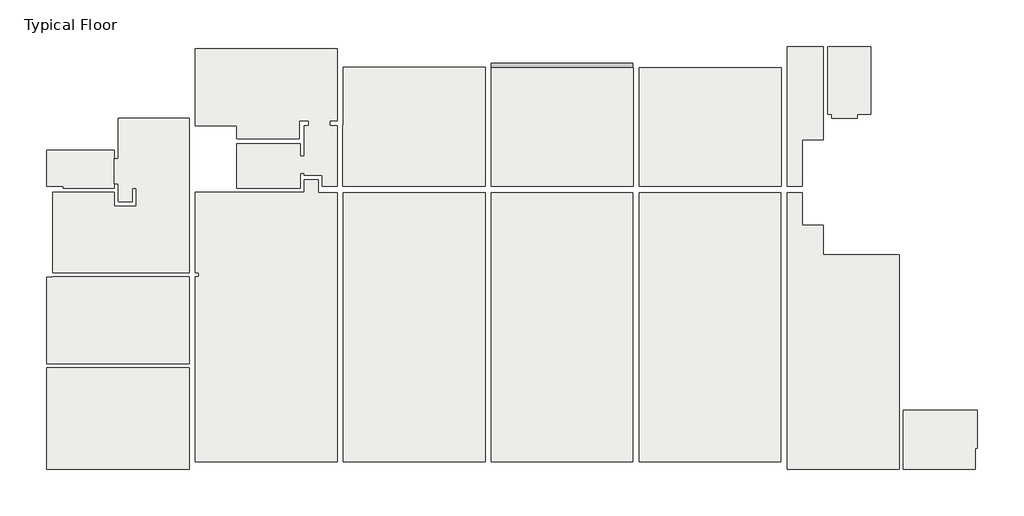
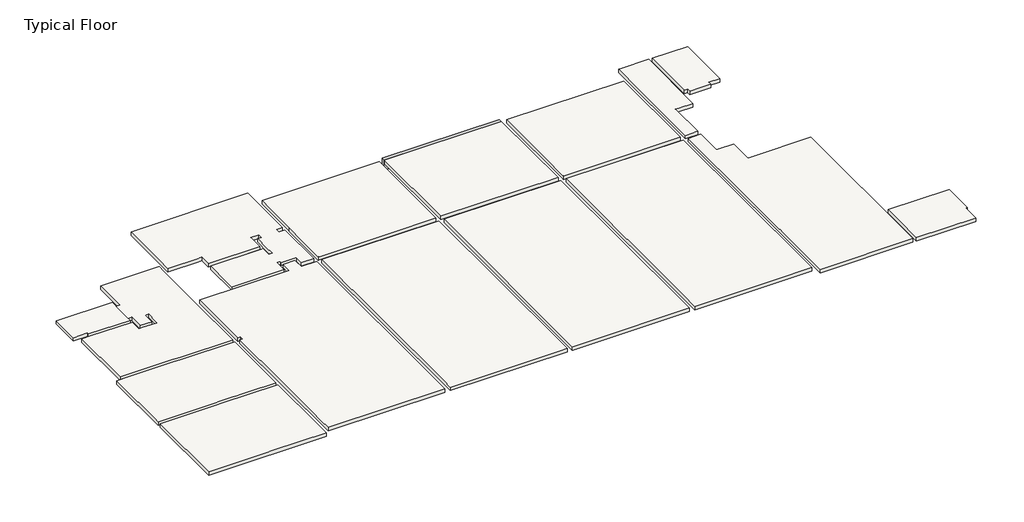
# One storey: 16 slabs, 1 beam.
"""IFC4 building model written with IfcOpenShell, lengths in millimetres."""

from ifc_helpers import new_model, si_unit, frame, origin, place, context, project, spatial, polyline, outline, extrude, faceted_brep, element, save

model = new_model("IFC4")

# Units and contexts
model_context = context("Model", 3, world=origin())
ifc_project = project(units=[si_unit("LENGTHUNIT", "METRE", prefix="MILLI")], contexts=[model_context])

# Site, building, storey
site = spatial("IfcSite", under=ifc_project)
building = spatial("IfcBuilding", under=site)
storey = spatial("IfcBuildingStorey", under=building, Name="Typical Floor", Elevation=4000.0)

# Beam
placement = place(None, origin())
element("IfcBeam", 1, ObjectType="Concrete Rectengular Beam : 20/60", at=placement, inside=storey, context=model_context, shape_type="Brep", body=[
    faceted_brep([(7056.7343244, 23405.5571184, 4000.0), (358.2285773, 23405.5571184, 4000.0), (358.2285773, 23210.5571184, 4000.0), (7056.7343244, 23210.5571184, 4000.0), (7056.7343244, 23405.5571184, 3400.0), (358.2285773, 23405.5571184, 3400.0), (7056.7343244, 23205.5571184, 3400.0), (358.2285773, 23205.5571184, 3400.0), (7056.7343244, 23205.5571184, 3790.0), (358.2285773, 23205.5571184, 3790.0), (7056.7343244, 23210.5571184, 3790.0), (7056.7343244, 23206.5724441, 3790.0), (358.2285773, 23206.5724441, 3790.0), (358.2285773, 23210.5571184, 3790.0)], [[[0, 1, 2, 3]], [[0, 4, 5, 1]], [[4, 6, 7, 5]], [[7, 6, 8, 9]], [[4, 0, 3, 10, 11, 8, 6]], [[1, 5, 7, 9, 12, 13, 2]], [[10, 13, 12, 9, 8, 11]], [[13, 10, 3, 2]]]),
])

# Slabs
element("IfcSlab", 2, ObjectType="21", at=placement, inside=storey, context=model_context, shape_type="Brep", body=[
    faceted_brep([(-6644.3384725, 23225.5571184, 3790.0), (58.2285773, 23225.5571184, 3790.0), (58.2285773, 23206.5724441, 3790.0), (68.2285773, 23206.5724441, 3790.0), (68.2285773, 17597.4228975, 3790.0), (58.2285773, 17597.4228975, 3790.0), (58.2285773, 17587.4228975, 3790.0), (-6644.3384725, 17587.4228975, 3790.0), (-6644.3384725, 17597.4228975, 3790.0), (-6674.3384725, 17597.4228975, 3790.0), (-6674.3384725, 20454.6567352, 3790.0), (-6644.3384725, 20454.6567352, 3790.0), (-6644.3384725, 23205.5571184, 3790.0), (58.2285773, 23225.5571184, 4000.0), (-6644.3384725, 23225.5571184, 4000.0), (-6644.3384725, 20704.6567352, 4000.0), (-6644.3384725, 20454.6567352, 4000.0), (-6674.3384725, 20454.6567352, 4000.0), (-6674.3384725, 17597.4228975, 4000.0), (-6644.3384725, 17597.4228975, 4000.0), (-6644.3384725, 17587.4228975, 4000.0), (58.2285773, 17587.4228975, 4000.0), (58.2285773, 17597.4228975, 4000.0), (68.2285773, 17597.4228975, 4000.0), (68.2285773, 23206.5724441, 4000.0), (58.2285773, 23206.5724441, 4000.0)], [[[0, 1, 2, 3, 4, 5, 6, 7, 8, 9, 10, 11, 12]], [[13, 14, 15, 16, 17, 18, 19, 20, 21, 22, 23, 24, 25]], [[3, 24, 23, 4]], [[6, 21, 20, 7]], [[17, 10, 9, 18]], [[0, 14, 13, 1]], [[14, 0, 12, 11, 16, 15]], [[2, 25, 24, 3]], [[25, 2, 1, 13]], [[5, 22, 21, 6]], [[22, 5, 4, 23]], [[16, 11, 10, 17]], [[8, 19, 18, 9]], [[19, 8, 7, 20]]]),
])
element("IfcSlab", 3, ObjectType="21", at=placement, inside=storey, context=model_context, shape_type="Brep", body=[
    faceted_brep([(7061.7343244, 17597.4228975, 3790.0), (7056.7343244, 17597.4228975, 3790.0), (358.2285773, 17597.4228975, 3790.0), (353.2285773, 17597.4228975, 3790.0), (353.2285773, 23206.5724441, 3790.0), (358.2285773, 23206.5724441, 3790.0), (358.2285773, 23210.5571184, 3790.0), (7056.7343244, 23210.5571184, 3790.0), (7056.7343244, 23206.5724441, 3790.0), (7061.7343244, 23206.5724441, 3790.0), (353.2285773, 17597.4228975, 4000.0), (358.2285773, 17597.4228975, 4000.0), (7056.7343244, 17597.4228975, 4000.0), (7061.7343244, 17597.4228975, 4000.0), (7061.7343244, 23206.5724441, 4000.0), (7056.7343244, 23206.5724441, 4000.0), (7056.7343244, 23210.5571184, 4000.0), (358.2285773, 23210.5571184, 4000.0), (358.2285773, 23206.5724441, 4000.0), (353.2285773, 23206.5724441, 4000.0)], [[[0, 1, 2, 3, 4, 5, 6, 7, 8, 9]], [[10, 11, 12, 13, 14, 15, 16, 17, 18, 19]], [[13, 0, 9, 14]], [[3, 2, 1, 0, 13, 12, 11, 10]], [[3, 10, 19, 4]], [[6, 17, 16, 7]], [[5, 18, 17, 6]], [[18, 5, 4, 19]], [[8, 15, 14, 9]], [[15, 8, 7, 16]]]),
])
element("IfcSlab", 4, ObjectType="21", at=placement, inside=storey, context=model_context, shape_type="Brep", body=[
    faceted_brep([(7356.7343244, 23206.5724441, 3790.0), (7356.7343244, 23210.5571184, 3790.0), (14058.5350907, 23210.5571184, 3790.0), (14058.5350907, 23206.5724441, 3790.0), (14063.5350907, 23206.5724441, 3790.0), (14063.5350907, 23205.5571184, 3790.0), (14063.5350907, 17597.4228975, 3790.0), (14058.5350907, 17597.4228975, 3790.0), (14058.5350907, 17587.4228975, 3790.0), (7356.7343244, 17587.4228975, 3790.0), (7356.7343244, 17597.4228975, 3790.0), (7351.7343244, 17597.4228975, 3790.0), (7351.7343244, 23206.5724441, 3790.0), (7356.7343244, 23210.5571184, 4000.0), (7356.7343244, 23206.5724441, 4000.0), (7351.7343244, 23206.5724441, 4000.0), (7351.7343244, 17597.4228975, 4000.0), (7356.7343244, 17597.4228975, 4000.0), (7356.7343244, 17587.4228975, 4000.0), (14058.5350907, 17587.4228975, 4000.0), (14058.5350907, 17597.4228975, 4000.0), (14063.5350907, 17597.4228975, 4000.0), (14063.5350907, 23205.5571184, 4000.0), (14063.5350907, 23206.5724441, 4000.0), (14058.5350907, 23206.5724441, 4000.0), (14058.5350907, 23210.5571184, 4000.0)], [[[0, 1, 2, 3, 4, 5, 6, 7, 8, 9, 10, 11, 12]], [[13, 14, 15, 16, 17, 18, 19, 20, 21, 22, 23, 24, 25]], [[4, 23, 22, 21, 6, 5]], [[18, 9, 8, 19]], [[15, 12, 11, 16]], [[1, 13, 25, 2]], [[0, 14, 13, 1]], [[14, 0, 12, 15]], [[17, 10, 9, 18]], [[10, 17, 16, 11]], [[24, 3, 2, 25]], [[3, 24, 23, 4]], [[20, 7, 6, 21]], [[7, 20, 19, 8]]]),
])
element("IfcSlab", 5, ObjectType="21", at=placement, inside=storey, context=model_context, shape_type="Brep", body=[
    faceted_brep([(14058.5350907, 17297.4228975, 3790.0), (14058.5350907, 4552.8176548, 3790.0), (7356.7343244, 4552.8176548, 3790.0), (7356.7343244, 17297.4228975, 3790.0), (14058.5350907, 17297.4228975, 4000.0), (7356.7343244, 17297.4228975, 4000.0), (7356.7343244, 5204.8099919, 4000.0), (7356.7343244, 4552.8176548, 4000.0), (14058.5350907, 4552.8176548, 4000.0), (14058.5350907, 5204.8099919, 4000.0)], [[[0, 1, 2, 3]], [[4, 5, 6, 7, 8, 9]], [[1, 0, 4, 9, 8]], [[2, 1, 8, 7]], [[3, 2, 7, 6, 5]], [[0, 3, 5, 4]]]),
])
element("IfcSlab", 6, ObjectType="21", at=placement, inside=storey, context=model_context, shape_type="Brep", body=[
    faceted_brep([(7056.7343244, 17297.4228975, 3790.0), (7056.7343244, 4552.8176548, 3790.0), (358.2285773, 4552.8176548, 3790.0), (358.2285773, 17297.4228975, 3790.0), (7056.7343244, 17297.4228975, 4000.0), (358.2285773, 17297.4228975, 4000.0), (358.2285773, 5204.8099919, 4000.0), (358.2285773, 4552.8176548, 4000.0), (7056.7343244, 4552.8176548, 4000.0), (7056.7343244, 5204.8099919, 4000.0)], [[[0, 1, 2, 3]], [[4, 5, 6, 7, 8, 9]], [[1, 0, 4, 9, 8]], [[2, 1, 8, 7]], [[3, 2, 7, 6, 5]], [[0, 3, 5, 4]]]),
])
element("IfcSlab", 7, ObjectType="21", at=placement, inside=storey, context=model_context, shape_type="Brep", body=[
    faceted_brep([(58.2285773, 17297.4228975, 3790.0), (58.2285773, 4552.8176548, 3790.0), (-6644.3384725, 4552.8176548, 3790.0), (-6644.3384725, 17297.4228975, 3790.0), (58.2285773, 17297.4228975, 4000.0), (-6644.3384725, 17297.4228975, 4000.0), (-6644.3384725, 5204.8099919, 4000.0), (-6644.3384725, 4552.8176548, 4000.0), (58.2285773, 4552.8176548, 4000.0), (58.2285773, 5204.8099919, 4000.0)], [[[0, 1, 2, 3]], [[4, 5, 6, 7, 8, 9]], [[1, 0, 4, 9, 8]], [[2, 1, 8, 7]], [[3, 2, 7, 6, 5]], [[0, 3, 5, 4]]]),
])
element("IfcSlab", 8, ObjectType="21", at=placement, inside=storey, context=model_context, shape_type="Brep", body=[
    faceted_brep([(-13943.2656756, 9206.6873866, 3790.0), (-20690.7944112, 9206.6873866, 3790.0), (-20690.7944112, 13148.3800933, 3790.0), (-20690.7944112, 13298.3800933, 3790.0), (-20386.1465057, 13298.5145478, 3790.0), (-20386.1465057, 13303.9096088, 3790.0), (-20386.1465057, 13308.9096088, 3790.0), (-17368.3423039, 13308.9096088, 3790.0), (-17368.3423039, 13303.9096088, 3790.0), (-16968.3423039, 13303.9096088, 3790.0), (-16968.3423039, 13308.9096088, 3790.0), (-13944.4917292, 13308.9096088, 3790.0), (-13944.4917292, 13303.9096088, 3790.0), (-13943.2656756, 13303.9096088, 3790.0), (-20690.7944112, 9206.6873866, 4000.0), (-20678.0944112, 9206.6873866, 4000.0), (-17516.5223806, 9206.6873866, 4000.0), (-17116.5223806, 9206.6873866, 4000.0), (-13943.2656756, 9206.6873866, 4000.0), (-13943.2656756, 13303.9096088, 4000.0), (-13944.4917292, 13303.9096088, 4000.0), (-13944.4917292, 13308.9096088, 4000.0), (-16968.3423039, 13308.9096088, 4000.0), (-16968.3423039, 13303.9096088, 4000.0), (-17368.3423039, 13303.9096088, 4000.0), (-17368.3423039, 13308.9096088, 4000.0), (-20386.1465057, 13308.9096088, 4000.0), (-20386.1465057, 13298.5145478, 4000.0), (-20540.7944404, 13298.4462949, 4000.0), (-20690.7944112, 13298.3800933, 4000.0), (-20690.7944112, 13148.3800933, 4000.0)], [[[0, 1, 2, 3, 4, 5, 6, 7, 8, 9, 10, 11, 12, 13]], [[14, 15, 16, 17, 18, 19, 20, 21, 22, 23, 24, 25, 26, 27, 28, 29, 30]], [[18, 0, 13, 19]], [[1, 0, 18, 17, 16, 15, 14]], [[1, 14, 30, 29, 3, 2]], [[6, 26, 25, 7]], [[10, 22, 21, 11]], [[3, 29, 28, 27, 4]], [[4, 27, 26, 6, 5]], [[9, 23, 22, 10]], [[23, 9, 8, 24]], [[24, 8, 7, 25]], [[12, 20, 19, 13]], [[20, 12, 11, 21]]]),
])
element("IfcSlab", 9, ObjectType="21", at=placement, inside=storey, context=model_context, shape_type="Brep", body=[
    faceted_brep([(-13943.2656756, 9006.6873866, 3790.0), (-13943.2656756, 4206.6682295, 3790.0), (-20492.8250626, 4206.6682295, 3790.0), (-20690.7944112, 4206.6682295, 3790.0), (-20690.7944112, 9006.6873866, 3790.0), (-13943.2656756, 4206.6682295, 4000.0), (-13943.2656756, 5204.8099919, 4000.0), (-13943.2656756, 9006.6873866, 4000.0), (-17116.5223806, 9006.6873866, 4000.0), (-17516.5223806, 9006.6873866, 4000.0), (-20678.0944112, 9006.6873866, 4000.0), (-20690.7944112, 9006.6873866, 4000.0), (-20690.7944112, 8705.6720609, 4000.0), (-20690.7944112, 4206.6682295, 4000.0), (-20492.8250626, 4206.6682295, 4000.0), (-17416.9438365, 4206.6682295, 4000.0), (-17016.9438365, 4206.6682295, 4000.0)], [[[0, 1, 2, 3, 4]], [[5, 6, 7, 8, 9, 10, 11, 12, 13, 14, 15, 16]], [[1, 0, 7, 6, 5]], [[1, 5, 16, 15, 14, 13, 3, 2]], [[4, 3, 13, 12, 11]], [[0, 4, 11, 10, 9, 8, 7]]]),
])
element("IfcSlab", 10, ObjectType="21", at=placement, inside=storey, context=model_context, shape_type="Brep", body=[
    faceted_brep([(-8494.4725721, 17905.9594172, 3790.0), (-7834.4725721, 17905.9594172, 3790.0), (-7834.4725721, 17297.4228975, 3790.0), (-7634.4725721, 17297.4228975, 3790.0), (-6944.3384725, 17297.4228975, 3790.0), (-6944.3384725, 4552.8176548, 3790.0), (-13643.2656756, 4552.8176548, 3790.0), (-13643.2656756, 13303.9096088, 3790.0), (-13494.4917292, 13303.9096088, 3790.0), (-13494.4917292, 13503.9096088, 3790.0), (-13643.2656756, 13503.9096088, 3790.0), (-13643.2656756, 17304.7716778, 3790.0), (-8494.4725721, 17304.7716778, 3790.0), (-8494.4725721, 17504.7716778, 3790.0), (-7834.4725721, 17905.9594172, 4000.0), (-8494.4725721, 17905.9594172, 4000.0), (-8494.4725721, 17504.7716778, 4000.0), (-8494.4725721, 17304.7716778, 4000.0), (-13643.2656756, 17304.7716778, 4000.0), (-13643.2656756, 13503.9096088, 4000.0), (-13494.4917292, 13503.9096088, 4000.0), (-13494.4917292, 13303.9096088, 4000.0), (-13643.2656756, 13303.9096088, 4000.0), (-13643.2656756, 9206.6873866, 4000.0), (-13643.2656756, 9006.6873866, 4000.0), (-13643.2656756, 5204.8099919, 4000.0), (-13643.2656756, 4552.8176548, 4000.0), (-6944.3384725, 4552.8176548, 4000.0), (-6944.3384725, 5204.8099919, 4000.0), (-6944.3384725, 17297.4228975, 4000.0), (-7634.4725721, 17297.4228975, 4000.0), (-7834.4725721, 17297.4228975, 4000.0)], [[[0, 1, 2, 3, 4, 5, 6, 7, 8, 9, 10, 11, 12, 13]], [[14, 15, 16, 17, 18, 19, 20, 21, 22, 23, 24, 25, 26, 27, 28, 29, 30, 31]], [[15, 0, 13, 12, 17, 16]], [[1, 0, 15, 14]], [[2, 1, 14, 31]], [[2, 31, 30, 29, 4, 3]], [[5, 4, 29, 28, 27]], [[6, 5, 27, 26]], [[7, 6, 26, 25, 24, 23, 22]], [[8, 7, 22, 21]], [[9, 8, 21, 20]], [[10, 9, 20, 19]], [[11, 10, 19, 18]], [[12, 11, 18, 17]]]),
])
element("IfcSlab", 11, ObjectType="21", at=placement, inside=storey, context=model_context, shape_type="Brep", body=[
    faceted_brep([(-8685.7944112, 19594.6567352, 3790.0), (-8685.7944112, 19006.7257008, 3790.0), (-8485.7944112, 19006.7257008, 3790.0), (-8485.7944112, 19594.6567352, 3790.0), (-8485.7944112, 20454.6567352, 3790.0), (-8291.2541813, 20454.6567352, 3790.0), (-8291.2541813, 20704.6567352, 3790.0), (-8735.7944112, 20704.6567352, 3790.0), (-8735.7944112, 20454.6567352, 3790.0), (-8735.7944112, 19844.6567352, 3790.0), (-11690.9285108, 19844.6567352, 3790.0), (-11690.9285108, 20459.7142065, 3790.0), (-11890.9285108, 20459.7142065, 3790.0), (-13643.2656756, 20459.7142065, 3790.0), (-13643.2656756, 24104.7142065, 3790.0), (-6944.3384725, 24104.7142065, 3790.0), (-6944.3384725, 20704.6567352, 3790.0), (-7292.0970932, 20704.6567352, 3790.0), (-7292.0970932, 20454.6567352, 3790.0), (-6944.3384725, 20454.6567352, 3790.0), (-6944.3384725, 17597.4228975, 3790.0), (-7634.4725721, 17597.4228975, 3790.0), (-7634.4725721, 17905.9594172, 3790.0), (-7634.4725721, 18105.9594172, 3790.0), (-8494.4725721, 18105.9594172, 3790.0), (-8494.4725721, 18206.553287, 3790.0), (-8694.4725721, 18206.553287, 3790.0), (-8694.4725721, 17504.7716778, 3790.0), (-11690.9285108, 17504.7716778, 3790.0), (-11690.9285108, 19594.6567352, 3790.0), (-8735.7944112, 19594.6567352, 3790.0), (-8685.7944112, 19006.7257008, 4000.0), (-8685.7944112, 19594.6567352, 4000.0), (-8735.7944112, 19594.6567352, 4000.0), (-11690.9285108, 19594.6567352, 4000.0), (-11690.9285108, 17504.7716778, 4000.0), (-8694.4725721, 17504.7716778, 4000.0), (-8694.4725721, 18206.553287, 4000.0), (-8494.4725721, 18206.553287, 4000.0), (-8494.4725721, 18105.9594172, 4000.0), (-7634.4725721, 18105.9594172, 4000.0), (-7634.4725721, 17905.9594172, 4000.0), (-7634.4725721, 17597.4228975, 4000.0), (-6944.3384725, 17597.4228975, 4000.0), (-6944.3384725, 20454.6567352, 4000.0), (-7292.0970932, 20454.6567352, 4000.0), (-7292.0970932, 20704.6567352, 4000.0), (-6944.3384725, 20704.6567352, 4000.0), (-6944.3384725, 24104.7142065, 4000.0), (-13643.2656756, 24104.7142065, 4000.0), (-13643.2656756, 20459.7142065, 4000.0), (-11890.9285108, 20459.7142065, 4000.0), (-11690.9285108, 20459.7142065, 4000.0), (-11690.9285108, 19844.6567352, 4000.0), (-8735.7944112, 19844.6567352, 4000.0), (-8735.7944112, 20454.6567352, 4000.0), (-8735.7944112, 20704.6567352, 4000.0), (-8291.2541813, 20704.6567352, 4000.0), (-8291.2541813, 20454.6567352, 4000.0), (-8485.7944112, 20454.6567352, 4000.0), (-8485.7944112, 19594.6567352, 4000.0), (-8485.7944112, 19006.7257008, 4000.0)], [[[0, 1, 2, 3, 4, 5, 6, 7, 8, 9, 10, 11, 12, 13, 14, 15, 16, 17, 18, 19, 20, 21, 22, 23, 24, 25, 26, 27, 28, 29, 30]], [[31, 32, 33, 34, 35, 36, 37, 38, 39, 40, 41, 42, 43, 44, 45, 46, 47, 48, 49, 50, 51, 52, 53, 54, 55, 56, 57, 58, 59, 60, 61]], [[32, 0, 30, 29, 34, 33]], [[1, 0, 32, 31]], [[2, 1, 31, 61]], [[2, 61, 60, 59, 4, 3]], [[5, 4, 59, 58]], [[6, 5, 58, 57]], [[7, 6, 57, 56]], [[7, 56, 55, 54, 9, 8]], [[10, 9, 54, 53]], [[11, 10, 53, 52]], [[11, 52, 51, 50, 13, 12]], [[14, 13, 50, 49]], [[15, 14, 49, 48]], [[16, 15, 48, 47]], [[17, 16, 47, 46]], [[18, 17, 46, 45]], [[19, 18, 45, 44]], [[20, 19, 44, 43]], [[21, 20, 43, 42]], [[21, 42, 41, 40, 23, 22]], [[24, 23, 40, 39]], [[25, 24, 39, 38]], [[26, 25, 38, 37]], [[27, 26, 37, 36]], [[28, 27, 36, 35]], [[29, 28, 35, 34]]]),
])
element("IfcSlab", 12, ObjectType="21", at=placement, inside=storey, context=model_context, shape_type="Brep", body=[
    faceted_brep([(-17492.1354074, 18905.1165054, 3790.0), (-17292.1354074, 18905.1165054, 3790.0), (-17292.1354074, 20806.0552027, 3790.0), (-13943.2656756, 20806.0552027, 3790.0), (-13943.2656756, 13503.9096088, 3790.0), (-20386.1465057, 13503.9096088, 3790.0), (-20386.1465057, 17305.3655475, 3790.0), (-19891.6373231, 17305.3655475, 3790.0), (-19891.6373231, 17304.7716778, 3790.0), (-17492.1354074, 17304.7716778, 3790.0), (-17492.1354074, 16652.7793406, 3790.0), (-17292.1354074, 16652.7793406, 3790.0), (-16441.1583959, 16652.7793406, 3790.0), (-16441.1583959, 16852.7793406, 3790.0), (-16441.1583959, 17503.7563521, 3790.0), (-16641.1583959, 17503.7563521, 3790.0), (-16641.1583959, 16852.7793406, 3790.0), (-17292.1354074, 16852.7793406, 3790.0), (-17292.1354074, 17706.9747429, 3790.0), (-17492.1354074, 17706.9747429, 3790.0), (-17292.1354074, 18905.1165054, 4000.0), (-17492.1354074, 18905.1165054, 4000.0), (-17492.1354074, 17706.9747429, 4000.0), (-17292.1354074, 17706.9747429, 4000.0), (-17292.1354074, 16852.7793406, 4000.0), (-16641.1583959, 16852.7793406, 4000.0), (-16641.1583959, 17503.7563521, 4000.0), (-16441.1583959, 17503.7563521, 4000.0), (-16441.1583959, 16852.7793406, 4000.0), (-16441.1583959, 16652.7793406, 4000.0), (-17292.1354074, 16652.7793406, 4000.0), (-17492.1354074, 16652.7793406, 4000.0), (-17492.1354074, 17304.7716778, 4000.0), (-19891.6373231, 17304.7716778, 4000.0), (-19891.6373231, 17305.3655475, 4000.0), (-20386.1465057, 17305.3655475, 4000.0), (-20386.1465057, 13648.5145478, 4000.0), (-20386.1465057, 13503.9096088, 4000.0), (-17368.3423039, 13503.9096088, 4000.0), (-16968.3423039, 13503.9096088, 4000.0), (-13944.4917292, 13503.9096088, 4000.0), (-13943.2656756, 13503.9096088, 4000.0), (-13943.2656756, 17304.7716778, 4000.0), (-13943.2656756, 20334.7142065, 4000.0), (-13943.2656756, 20806.0552027, 4000.0), (-17292.1354074, 20806.0552027, 4000.0)], [[[0, 1, 2, 3, 4, 5, 6, 7, 8, 9, 10, 11, 12, 13, 14, 15, 16, 17, 18, 19]], [[20, 21, 22, 23, 24, 25, 26, 27, 28, 29, 30, 31, 32, 33, 34, 35, 36, 37, 38, 39, 40, 41, 42, 43, 44, 45]], [[1, 0, 21, 20]], [[2, 1, 20, 45]], [[3, 2, 45, 44]], [[4, 3, 44, 43, 42, 41]], [[5, 4, 41, 40, 39, 38, 37]], [[6, 5, 37, 36, 35]], [[6, 35, 34, 7]], [[31, 10, 9, 32]], [[10, 31, 30, 29, 12, 11]], [[12, 29, 28, 27, 14, 13]], [[15, 14, 27, 26]], [[16, 15, 26, 25]], [[17, 16, 25, 24]], [[18, 17, 24, 23]], [[19, 18, 23, 22]], [[0, 19, 22, 21]], [[8, 33, 32, 9]], [[33, 8, 7, 34]]]),
])
element("IfcSlab", 13, ObjectType="21", at=placement, inside=storey, context=model_context, shape_type="Brep", body=[
    faceted_brep([(15057.6921788, 17597.4228975, 3790.0), (14358.5350907, 17597.4228975, 3790.0), (14358.5350907, 24204.7142065, 3790.0), (14464.3013742, 24204.7142065, 3790.0), (16064.3013742, 24204.7142065, 3790.0), (16064.3013742, 19803.6797237, 3790.0), (15257.6921788, 19803.6797237, 3790.0), (15057.6921788, 19803.6797237, 3790.0), (14358.5350907, 17597.4228975, 4000.0), (15057.6921788, 17597.4228975, 4000.0), (15057.6921788, 19803.6797237, 4000.0), (15257.6921788, 19803.6797237, 4000.0), (16064.3013742, 19803.6797237, 4000.0), (16064.3013742, 24204.7142065, 4000.0), (14464.3013742, 24204.7142065, 4000.0), (14358.5350907, 24204.7142065, 4000.0), (14358.5350907, 23206.5724441, 4000.0), (14358.5350907, 23205.5571184, 4000.0)], [[[0, 1, 2, 3, 4, 5, 6, 7]], [[8, 9, 10, 11, 12, 13, 14, 15, 16, 17]], [[1, 0, 9, 8]], [[2, 1, 8, 17, 16, 15]], [[3, 2, 15, 14]], [[4, 3, 14, 13]], [[5, 4, 13, 12]], [[5, 12, 11, 10, 7, 6]], [[0, 7, 10, 9]]]),
])
element("IfcSlab", 14, ObjectType="21", at=placement, inside=storey, context=model_context, shape_type="Brep", body=[
    faceted_brep([(16459.0523321, 21006.0552027, 3790.0), (16264.3013742, 21006.0552027, 3790.0), (16264.3013742, 24204.7142065, 3790.0), (18304.3013742, 24204.7142065, 3790.0), (18304.3013742, 21004.7142065, 3790.0), (17668.5350907, 21004.7142065, 3790.0), (17668.5350907, 20804.7142065, 3790.0), (16459.0523321, 20804.7142065, 3790.0), (16459.0523321, 20806.0552027, 3790.0), (16264.3013742, 21006.0552027, 4000.0), (16459.0523321, 21006.0552027, 4000.0), (16459.0523321, 20806.0552027, 4000.0), (16459.0523321, 20804.7142065, 4000.0), (17668.5350907, 20804.7142065, 4000.0), (17668.5350907, 21004.7142065, 4000.0), (18304.3013742, 21004.7142065, 4000.0), (18304.3013742, 24204.7142065, 4000.0), (16264.3013742, 24204.7142065, 4000.0)], [[[0, 1, 2, 3, 4, 5, 6, 7, 8]], [[9, 10, 11, 12, 13, 14, 15, 16, 17]], [[1, 0, 10, 9]], [[2, 1, 9, 17]], [[3, 2, 17, 16]], [[4, 3, 16, 15]], [[5, 4, 15, 14]], [[6, 5, 14, 13]], [[7, 6, 13, 12]], [[7, 12, 11, 10, 0, 8]]]),
])
element("IfcSlab", 15, ObjectType="21", at=placement, inside=storey, context=model_context, shape_type="Brep", body=[
    faceted_brep([(15057.6921788, 17297.4228975, 3790.0), (15057.6921788, 15755.2314479, 3790.0), (15257.6921788, 15755.2314479, 3790.0), (16056.849267, 15755.2314479, 3790.0), (16056.849267, 14353.8712946, 3790.0), (16256.849267, 14353.8712946, 3790.0), (19658.7266616, 14353.8712946, 3790.0), (19658.7266616, 4204.8099919, 3790.0), (14358.5350907, 4204.8099919, 3790.0), (14358.5350907, 17297.4228975, 3790.0), (15057.6921788, 15755.2314479, 4000.0), (15057.6921788, 17297.4228975, 4000.0), (14358.5350907, 17297.4228975, 4000.0), (14358.5350907, 5204.8099919, 4000.0), (14358.5350907, 4204.8099919, 4000.0), (19658.7266616, 4204.8099919, 4000.0), (19658.7266616, 14353.8712946, 4000.0), (16256.849267, 14353.8712946, 4000.0), (16056.849267, 14353.8712946, 4000.0), (16056.849267, 15755.2314479, 4000.0), (15257.6921788, 15755.2314479, 4000.0)], [[[0, 1, 2, 3, 4, 5, 6, 7, 8, 9]], [[10, 11, 12, 13, 14, 15, 16, 17, 18, 19, 20]], [[1, 0, 11, 10]], [[1, 10, 20, 19, 3, 2]], [[4, 3, 19, 18]], [[4, 18, 17, 16, 6, 5]], [[7, 6, 16, 15]], [[8, 7, 15, 14]], [[9, 8, 14, 13, 12]], [[0, 9, 12, 11]]]),
])
element("IfcSlab", 16, ObjectType="21", at=placement, inside=storey, context=model_context, shape_type="SweptSolid", body=[
    extrude(outline(polyline([(23358.9948608, 7004.1394939), (23358.9948608, 5204.1394939), (23258.9948608, 5204.1394939), (23258.9948608, 4204.8099919), (19858.7266616, 4204.8099919), (19858.7266616, 7004.1394939), (23358.9948608, 7004.1394939)])), frame((0.0, 0.0, 3790.0), z_axis=(0.0, 0.0, 1.0), x_axis=(1.0, 0.0, 0.0)), (0.0, 0.0, 1.0), 210.0),
])
element("IfcSlab", 17, ObjectType="21", at=placement, inside=storey, context=model_context, shape_type="Brep", body=[
    faceted_brep([(-17492.1354074, 17504.7716778, 3790.0), (-19891.6373231, 17504.7716778, 3790.0), (-19891.6373231, 17605.3655475, 3790.0), (-20690.7944112, 17605.3655475, 3790.0), (-20690.7944112, 19305.3655475, 3790.0), (-17492.1354074, 19305.3655475, 3790.0), (-17492.1354074, 18905.1165054, 3790.0), (-17492.1354074, 17706.9747429, 3790.0), (-19891.6373231, 17504.7716778, 4000.0), (-17492.1354074, 17504.7716778, 4000.0), (-17492.1354074, 17706.9747429, 4000.0), (-17492.1354074, 18905.1165054, 4000.0), (-17492.1354074, 19305.3655475, 4000.0), (-20690.7944112, 19305.3655475, 4000.0), (-20690.7944112, 17605.3655475, 4000.0), (-19891.6373231, 17605.3655475, 4000.0)], [[[0, 1, 2, 3, 4, 5, 6, 7]], [[8, 9, 10, 11, 12, 13, 14, 15]], [[9, 0, 7, 6, 5, 12, 11, 10]], [[1, 0, 9, 8]], [[2, 1, 8, 15]], [[3, 2, 15, 14]], [[4, 3, 14, 13]], [[5, 4, 13, 12]]]),
])

save(model, "model.ifc")

# Revit data of these elements
# Type "Concrete Rectengular Beam : 20/60"
#   Length [instance default] = 152.4 cm
#   b = 20 cm
#   h = 60 cm
#   Structural Material [instance default] = Concrete
#   Assembly Code = ""
# Type "21"
#   Function = 0
#   Layers, outside or top first: 21 cm "Concrete" (function 1)
# Element 1 (IfcBeam, "Concrete Rectengular Beam : 20/60")
#   Comments = ""
#   Mark = "B14"
#   SOFiSTiK_AMG_Comments = ""
#   SOFiSTiK_AMG_Scheduled = yes
#   SOFiSTiK_AMG_Adjusted = yes
#   Structural Material = Concrete
#   Phase Created = New Construction
#   Materials on its faces: "Concrete"
# Element 2 (IfcSlab, "21")
#   Mark = "S1"
#   SOFiSTiK_AMG_Comments = ""
#   Height Offset From Level = 0 cm
#   built-in parameter 1001954 = 1
#   SOFiSTiK_AMG_Scheduled = yes
#   SOFiSTiK_AMG_Adjusted = yes
#   Phase Created = New Construction
#   Materials on its faces: "Concrete"
# Element 3 (IfcSlab, "21")
#   Mark = "S2"
#   SOFiSTiK_AMG_Comments = ""
#   Height Offset From Level = 0 cm
#   built-in parameter 1001954 = 1
#   SOFiSTiK_AMG_Scheduled = yes
#   SOFiSTiK_AMG_Adjusted = yes
#   Phase Created = New Construction
#   Materials on its faces: "Concrete"
# Element 4 (IfcSlab, "21")
#   Mark = "S3"
#   SOFiSTiK_AMG_Comments = ""
#   Height Offset From Level = 0 cm
#   built-in parameter 1001954 = 1
#   SOFiSTiK_AMG_Scheduled = yes
#   SOFiSTiK_AMG_Adjusted = yes
#   Phase Created = New Construction
#   Materials on its faces: "Concrete"
# Element 5 (IfcSlab, "21")
#   Mark = "S4"
#   SOFiSTiK_AMG_Comments = ""
#   Height Offset From Level = 0 cm
#   built-in parameter 1001954 = 1
#   SOFiSTiK_AMG_Scheduled = yes
#   SOFiSTiK_AMG_Adjusted = yes
#   Phase Created = New Construction
#   Materials on its faces: "Concrete"
# Element 6 (IfcSlab, "21")
#   Mark = "S5"
#   SOFiSTiK_AMG_Comments = ""
#   Height Offset From Level = 0 cm
#   built-in parameter 1001954 = 1
#   SOFiSTiK_AMG_Scheduled = yes
#   SOFiSTiK_AMG_Adjusted = yes
#   Phase Created = New Construction
#   Materials on its faces: "Concrete"
# Element 7 (IfcSlab, "21")
#   Mark = "S6"
#   SOFiSTiK_AMG_Comments = ""
#   Height Offset From Level = 0 cm
#   built-in parameter 1001954 = 1
#   SOFiSTiK_AMG_Scheduled = yes
#   SOFiSTiK_AMG_Adjusted = yes
#   Phase Created = New Construction
#   Materials on its faces: "Concrete"
# Element 8 (IfcSlab, "21")
#   Mark = "S7"
#   SOFiSTiK_AMG_Comments = ""
#   Height Offset From Level = 0 cm
#   built-in parameter 1001954 = 1
#   SOFiSTiK_AMG_Scheduled = yes
#   SOFiSTiK_AMG_Adjusted = yes
#   Phase Created = New Construction
#   Materials on its faces: "Concrete"
# Element 9 (IfcSlab, "21")
#   Mark = "S8"
#   SOFiSTiK_AMG_Comments = ""
#   Height Offset From Level = 0 cm
#   built-in parameter 1001954 = 1
#   SOFiSTiK_AMG_Scheduled = yes
#   SOFiSTiK_AMG_Adjusted = yes
#   Phase Created = New Construction
#   Materials on its faces: "Concrete"
# Element 10 (IfcSlab, "21")
#   Mark = "S9"
#   SOFiSTiK_AMG_Comments = ""
#   Height Offset From Level = 0 cm
#   built-in parameter 1001954 = 1
#   SOFiSTiK_AMG_Scheduled = yes
#   SOFiSTiK_AMG_Adjusted = yes
#   Phase Created = New Construction
#   Materials on its faces: "Concrete"
# Element 11 (IfcSlab, "21")
#   Mark = "S10"
#   SOFiSTiK_AMG_Comments = ""
#   built-in parameter 1001955 = 1.5708 (stored number, unit not read)
#   Height Offset From Level = 0 cm
#   built-in parameter 1001954 = 1
#   SOFiSTiK_AMG_Scheduled = yes
#   SOFiSTiK_AMG_Adjusted = yes
#   Phase Created = New Construction
#   Materials on its faces: "Concrete"
# Element 12 (IfcSlab, "21")
#   Mark = "S11"
#   SOFiSTiK_AMG_Comments = ""
#   built-in parameter 1001955 = 1.5708 (stored number, unit not read)
#   Height Offset From Level = 0 cm
#   built-in parameter 1001954 = 1
#   SOFiSTiK_AMG_Scheduled = yes
#   SOFiSTiK_AMG_Adjusted = yes
#   Phase Created = New Construction
#   Materials on its faces: "Concrete"
# Element 13 (IfcSlab, "21")
#   Mark = "S12"
#   SOFiSTiK_AMG_Comments = ""
#   Height Offset From Level = 0 cm
#   built-in parameter 1001954 = 1
#   SOFiSTiK_AMG_Scheduled = yes
#   SOFiSTiK_AMG_Adjusted = yes
#   Phase Created = New Construction
#   Materials on its faces: "Concrete"
# Element 14 (IfcSlab, "21")
#   Mark = "S13"
#   SOFiSTiK_AMG_Comments = ""
#   built-in parameter 1001955 = 1.5708 (stored number, unit not read)
#   Height Offset From Level = 0 cm
#   built-in parameter 1001954 = 1
#   SOFiSTiK_AMG_Scheduled = yes
#   SOFiSTiK_AMG_Adjusted = yes
#   Phase Created = New Construction
#   Materials on its faces: "Concrete"
# Element 15 (IfcSlab, "21")
#   Mark = "S14"
#   SOFiSTiK_AMG_Comments = ""
#   Height Offset From Level = 0 cm
#   built-in parameter 1001954 = 1
#   SOFiSTiK_AMG_Scheduled = yes
#   SOFiSTiK_AMG_Adjusted = yes
#   Phase Created = New Construction
#   Materials on its faces: "Concrete"
# Element 16 (IfcSlab, "21")
#   Mark = "S15"
#   SOFiSTiK_AMG_Comments = ""
#   Height Offset From Level = 0 cm
#   built-in parameter 1001954 = 1
#   SOFiSTiK_AMG_Scheduled = yes
#   SOFiSTiK_AMG_Adjusted = yes
#   Phase Created = New Construction
#   Materials on its faces: "Concrete"
# Element 17 (IfcSlab, "21")
#   Mark = "S16"
#   SOFiSTiK_AMG_Comments = ""
#   Height Offset From Level = 0 cm
#   built-in parameter 1001954 = 1
#   SOFiSTiK_AMG_Scheduled = yes
#   SOFiSTiK_AMG_Adjusted = yes
#   Phase Created = New Construction
#   Materials on its faces: "Concrete"
# Materials
#   "Concrete": class "Concrete", colour RGB 192 192 192, transparency 0, Keynote = "01000", Description = "Cast-in-place concrete", Cost = 0
